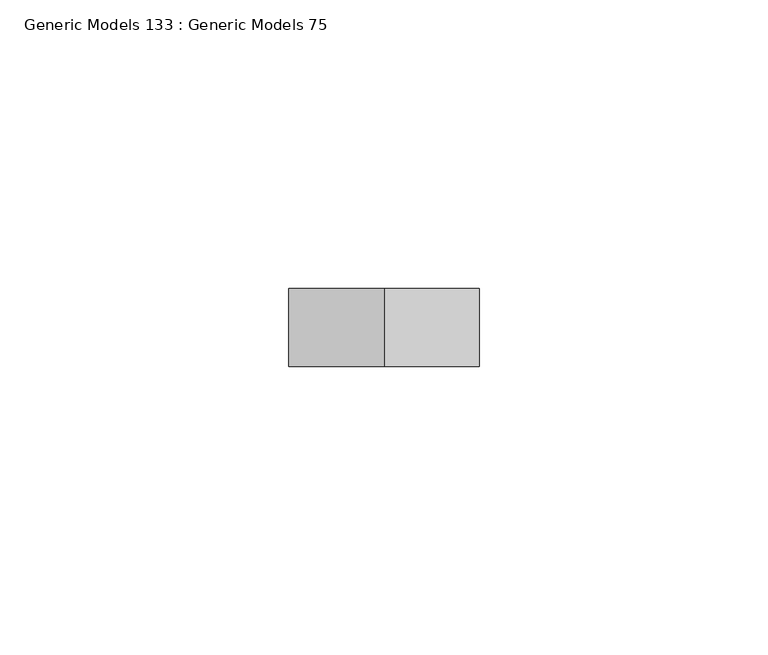
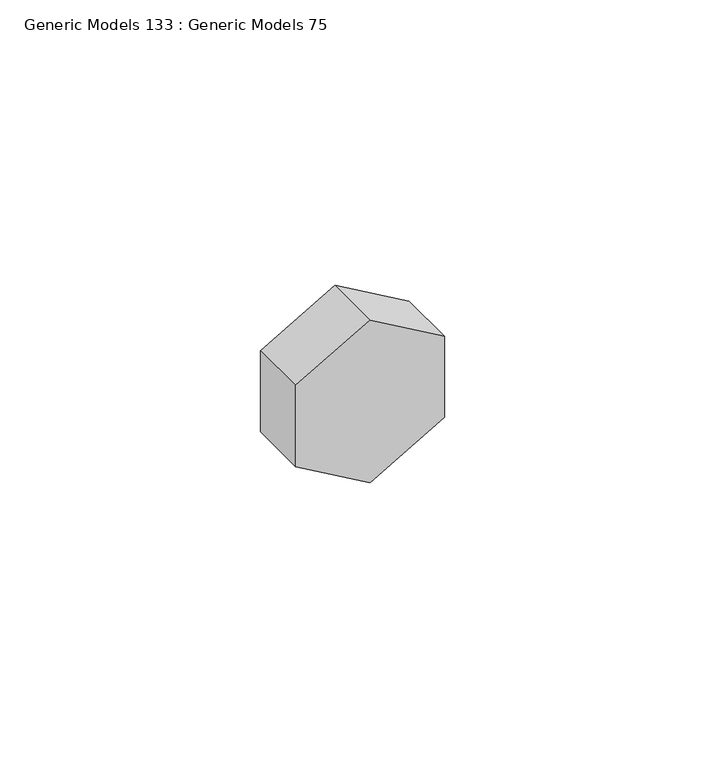
"""IFC4 building model written with IfcOpenShell, lengths in millimetres: proxy geometry, Generic Models 133 : Generic Models 75."""

import ifcopenshell
import ifcopenshell.guid

model = None  # the IFC model being written
_history = None  # IfcOwnerHistory: only IFC2X3 demands one
_inside = {}  # id of a spatial element -> (the spatial element, [elements in it])
_under = {}  # id of a project, library or spatial element -> (it, [spatial elements below it])
_declared = {}  # id of a project -> (the project, [libraries it declares])
_typed = {}  # id of a type object -> (the type object, [elements of that type])
_made_of = {}  # id of a material, layer set ... -> (it, [elements and type objects made of it])


def new_model(schema):
    """Start an empty IFC model of exactly this schema.

    Asked for "IFC4X3", IfcOpenShell would pick the latest addendum, in which some entities
    have other attributes; the version numbers below select the first issue.
    IFC2X3 requires an IfcOwnerHistory on every rooted entity: one is made here for all.
    """
    global model, _history
    if schema == "IFC4X3":
        model = ifcopenshell.file(schema_version=(4, 3, 0, 0))
    else:
        model = ifcopenshell.file(schema=schema)
    _inside.clear()
    _under.clear()
    _declared.clear()
    _typed.clear()
    _made_of.clear()
    _history = None
    if model.schema == "IFC2X3":
        org = make("IfcOrganization", Name="unknown")
        user = make(
            "IfcPersonAndOrganization",
            ThePerson=make("IfcPerson", FamilyName="unknown"),
            TheOrganization=org,
        )
        app = make(
            "IfcApplication",
            ApplicationDeveloper=org,
            Version="unknown",
            ApplicationFullName="unknown",
            ApplicationIdentifier="unknown",
        )
        _history = make(
            "IfcOwnerHistory",
            OwningUser=user,
            OwningApplication=app,
            ChangeAction="ADDED",
            CreationDate=0,
        )
    return model


def make(cls, **values):
    """One entity of the class cls with the attributes given. An attribute that is None is left unset."""
    return model.create_entity(
        cls, **{name: value for name, value in values.items() if value is not None}
    )


def rooted(cls, **values):
    """An entity with a GlobalId (a new one), such as an element, a storey or a relation."""
    return make(cls, GlobalId=ifcopenshell.guid.new(), OwnerHistory=_history, **values)


def si_unit(unit_type, name, prefix=None):
    """IfcSIUnit, for example si_unit("LENGTHUNIT", "METRE", prefix="MILLI")."""
    return make("IfcSIUnit", UnitType=unit_type, Prefix=prefix, Name=name)


def assignment(units):
    """IfcUnitAssignment: the units of a project."""
    return None if units is None else make("IfcUnitAssignment", Units=units)


def point(xyz):
    """IfcCartesianPoint."""
    return None if xyz is None else make("IfcCartesianPoint", Coordinates=xyz)


def direction(xyz):
    """IfcDirection."""
    return None if xyz is None else make("IfcDirection", DirectionRatios=xyz)


def frame(location, z_axis=None, x_axis=None):
    """IfcAxis2Placement3D, a coordinate frame: its origin and axes. An axis left out is left unset."""
    return make(
        "IfcAxis2Placement3D",
        Location=point(location),
        Axis=direction(z_axis),
        RefDirection=direction(x_axis),
    )


def origin():
    """The frame at (0, 0, 0) with its axes left unset."""
    return frame((0.0, 0.0, 0.0))


def place(relative_to, where):
    """IfcLocalPlacement: puts the frame where relative to a parent placement (None: the world)."""
    return make(
        "IfcLocalPlacement", PlacementRelTo=relative_to, RelativePlacement=where
    )


def context(
    kind, dimensions, precision=None, world=None, true_north=None, identifier=None
):
    """IfcGeometricRepresentationContext, for example the 3D "Model" context."""
    return make(
        "IfcGeometricRepresentationContext",
        ContextIdentifier=identifier,
        ContextType=kind,
        CoordinateSpaceDimension=dimensions,
        Precision=precision,
        WorldCoordinateSystem=world,
        TrueNorth=true_north,
    )


def project(units=None, contexts=None):
    """IfcProject with its units and contexts."""
    return rooted(
        "IfcProject",
        Name="project",
        RepresentationContexts=contexts,
        UnitsInContext=assignment(units),
    )


def spatial(cls, under=None, at=None, **own):
    """A site, building, storey or space (cls), placed at a placement, below another one or the project."""
    s = rooted(cls, ObjectPlacement=at, **own)
    if under is not None:
        _under.setdefault(under.id(), (under, []))[1].append(s)
    return s


def polyline(points):
    """IfcPolyline through the points."""
    return make("IfcPolyline", Points=[point(p) for p in points])


def outline(outer, holes=None, kind="AREA"):
    """IfcArbitraryClosedProfileDef: a profile drawn as a closed curve; with holes, ...WithVoids."""
    if holes is None:
        return make("IfcArbitraryClosedProfileDef", ProfileType=kind, OuterCurve=outer)
    return make(
        "IfcArbitraryProfileDefWithVoids",
        ProfileType=kind,
        OuterCurve=outer,
        InnerCurves=holes,
    )


def extrude(swept, where, along, depth):
    """IfcExtrudedAreaSolid: the profile swept, set in the frame where, extruded along a direction by depth."""
    return make(
        "IfcExtrudedAreaSolid",
        SweptArea=swept,
        Position=where,
        ExtrudedDirection=direction(along),
        Depth=depth,
    )


def shape(context_of_items, identifier, shape_type, items):
    """IfcShapeRepresentation: the items that make up one representation, for example the "Body"."""
    return make(
        "IfcShapeRepresentation",
        ContextOfItems=context_of_items,
        RepresentationIdentifier=identifier,
        RepresentationType=shape_type,
        Items=items,
    )


def source(mapping_origin, context_of_items, identifier, shape_type, items):
    """IfcRepresentationMap: a shape defined once, which mapped items show again and again."""
    return make(
        "IfcRepresentationMap",
        MappingOrigin=mapping_origin,
        MappedRepresentation=shape(context_of_items, identifier, shape_type, items),
    )


def transform(
    local_origin,
    x_axis=None,
    y_axis=None,
    z_axis=None,
    scale=None,
    scale2=None,
    scale3=None,
    uniform=True,
):
    """IfcCartesianTransformationOperator3D, or its non-uniform kind. x_axis, y_axis, z_axis: its Axis1, 2, 3."""
    if uniform:
        return make(
            "IfcCartesianTransformationOperator3D",
            Axis1=direction(x_axis),
            Axis2=direction(y_axis),
            LocalOrigin=point(local_origin),
            Scale=scale,
            Axis3=direction(z_axis),
        )
    return make(
        "IfcCartesianTransformationOperator3DnonUniform",
        Axis1=direction(x_axis),
        Axis2=direction(y_axis),
        LocalOrigin=point(local_origin),
        Scale=scale,
        Axis3=direction(z_axis),
        Scale2=scale2,
        Scale3=scale3,
    )


def mapped(mapping_source, mapping_target):
    """IfcMappedItem: shows the shape of a source again, moved by a transform."""
    return make(
        "IfcMappedItem", MappingSource=mapping_source, MappingTarget=mapping_target
    )


def made_of(thing, what):
    """Note that an element or type object is made of a material, layer set ...; save() writes the relation."""
    if what is not None:
        _made_of.setdefault(what.id(), (what, []))[1].append(thing)
    return thing


def element(
    cls,
    number,
    at=None,
    inside=None,
    cuts=None,
    type_object=None,
    material=None,
    context=None,
    identifier="Body",
    shape_type=None,
    held_by="IfcProductDefinitionShape",
    body=None,
    shapes=None,
    **own,
):
    """One element of the class cls, such as IfcWall. Its Tag is "e" and its number.

    at: its placement. inside: the storey or other place that contains it. cuts: it is an
    opening in that element (IfcRelVoidsElement). A single representation is given by context,
    identifier, shape_type and body (its items); several are given by shapes. held_by: the class
    of the entity that holds the representations. save() writes the other relations.
    """
    e = rooted(cls, Tag="e%d" % number, ObjectPlacement=at, **own)
    if body is not None:
        shapes = [shape(context, identifier, shape_type, body)]
    if shapes is not None:
        e.Representation = make(held_by, Representations=shapes)
    if inside is not None:
        _inside.setdefault(inside.id(), (inside, []))[1].append(e)
    if cuts is not None:
        rooted(
            "IfcRelVoidsElement", RelatingBuildingElement=cuts, RelatedOpeningElement=e
        )
    if type_object is not None:
        _typed.setdefault(type_object.id(), (type_object, []))[1].append(e)
    return made_of(e, material)


def aggregate(whole, parts):
    """IfcRelAggregates: a whole, such as a stair, and the parts it consists of."""
    return rooted("IfcRelAggregates", RelatingObject=whole, RelatedObjects=parts)


def save(model, path):
    """Write the relations noted so far, then the file.

    IfcRelAggregates (storeys below a building ...), IfcRelContainedInSpatialStructure (elements
    in a storey), IfcRelDefinesByType, IfcRelAssociatesMaterial and IfcRelDeclares: one each for
    every whole, place, type object, material and project.
    """
    for whole, parts in _under.values():
        aggregate(whole, parts)
    for where, things in _inside.values():
        rooted(
            "IfcRelContainedInSpatialStructure",
            RelatedElements=things,
            RelatingStructure=where,
        )
    for kind, things in _typed.values():
        rooted("IfcRelDefinesByType", RelatedObjects=things, RelatingType=kind)
    for what, things in _made_of.values():
        rooted("IfcRelAssociatesMaterial", RelatedObjects=things, RelatingMaterial=what)
    for by, libraries in _declared.values():
        rooted("IfcRelDeclares", RelatingContext=by, RelatedDefinitions=libraries)
    model.write(path)


def generic_models_133_generic_models_75_581e0cd9(model_context):
    return source(origin(), model_context, "Body", "SweptSolid", [
        extrude(outline(polyline([(268485.9375, 31991.9073871), (268504.9875, 31991.9073871), (268514.5125, 31975.4096032), (268504.9875, 31958.9118192), (268485.9375, 31958.9118192), (268476.4125, 31975.4096032), (268485.9375, 31991.9073871)])), frame((0.0, 34159.7273424, 0.0), z_axis=(0.0, 1.0, 0.0), x_axis=(0.0, 0.0, 1.0)), (0.0, 0.0, 1.0), 13.49375),
    ])


if __name__ == "__main__":
    model = new_model("IFC4")
    model_context = context("Model", 3, world=origin())
    ifc_project = project(units=[si_unit("LENGTHUNIT", "METRE", prefix="MILLI")], contexts=[model_context])
    site = spatial("IfcSite", under=ifc_project)
    building = spatial("IfcBuilding", under=site)
    placement = place(None, origin())
    generic_models_133_generic_models_75_shape = generic_models_133_generic_models_75_581e0cd9(model_context)
    element("IfcBuildingElementProxy", 1, Name="Generic Models 133 : Generic Models 75", ObjectType="Generic Models 133 : Generic Models 75", at=placement, inside=building, context=model_context, shape_type="MappedRepresentation", body=[
        mapped(generic_models_133_generic_models_75_shape, transform((0.0, 0.0, 0.0), x_axis=(1.0, 0.0, 0.0), y_axis=(0.0, 1.0, 0.0), z_axis=(0.0, 0.0, 1.0))),
    ])
    save(model, "model.ifc")
